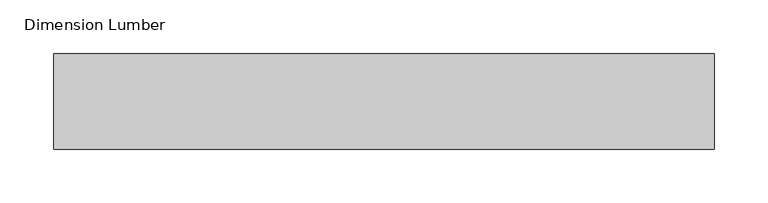
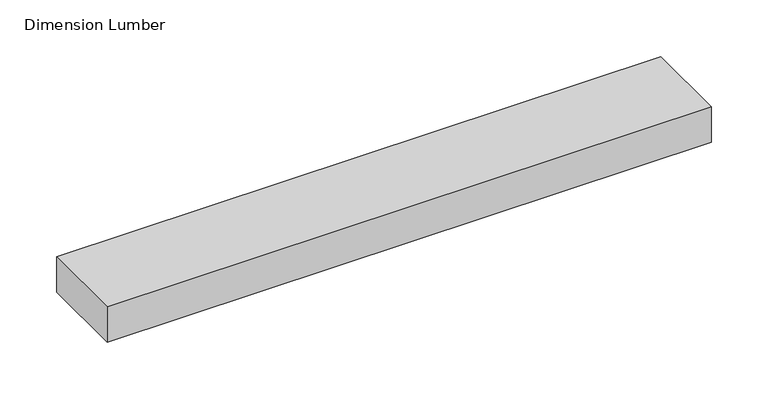
"""IFC4 building model written with IfcOpenShell, lengths in millimetres: beam geometry, Dimension Lumber : Top Supporting Lumbers."""

from ifc_helpers import new_model, si_unit, frame, origin, place, context, project, spatial, polyline, outline, extrude, source, transform, mapped, element, save


def dimension_lumber_5c8890d8(model_context):
    return source(origin(), model_context, "Body", "SweptSolid", [
        extrude(outline(polyline([(330.0062925, 44.45), (330.0062925, -44.45), (-285.5562925, -44.45), (-285.5562925, 44.45), (330.0062925, 44.45)])), frame((0.0, 0.0, -19.05), z_axis=(0.0, 0.0, 1.0), x_axis=(1.0, 0.0, 0.0)), (0.0, 0.0, 1.0), 38.1),
    ])


if __name__ == "__main__":
    model = new_model("IFC4")
    model_context = context("Model", 3, world=origin())
    ifc_project = project(units=[si_unit("LENGTHUNIT", "METRE", prefix="MILLI")], contexts=[model_context])
    site = spatial("IfcSite", under=ifc_project)
    building = spatial("IfcBuilding", under=site)
    placement = place(None, origin())
    dimension_lumber_shape = dimension_lumber_5c8890d8(model_context)
    element("IfcBeam", 1, ObjectType="Dimension Lumber : Top Supporting Lumbers", at=placement, inside=building, context=model_context, shape_type="MappedRepresentation", body=[
        mapped(dimension_lumber_shape, transform((0.0, 0.0, 0.0), x_axis=(1.0, 0.0, 0.0), y_axis=(0.0, 1.0, 0.0), z_axis=(0.0, 0.0, 1.0))),
    ])
    save(model, "model.ifc")

# Revit data of these elements
# Type "Dimension Lumber : Top Supporting Lumbers"
#   Assembly Code = "B10"
#   A = 0.0364583 SF
#   Length [instance default] = 5' - 0"
#   b = 0' - 3 1/2"
#   d = 0' - 1 1/2"
#   Structural Material [instance default] = Softwood, Lumber
# Element 1 (IfcBeam, "Dimension Lumber : Top Supporting Lumbers")
#   Structural Material = Douglas Fir #2
#   Materials on its faces: "Douglas Fir #2"
# Materials
#   "Softwood, Lumber": class "Wood", colour RGB 223 192 134, transparency 0, Description = "Pinus Echinata", Cost = 0
#   "Douglas Fir #2": class "Wood", colour RGB 223 192 134, transparency 0, Description = "Pinus Echinata", Cost = 0
